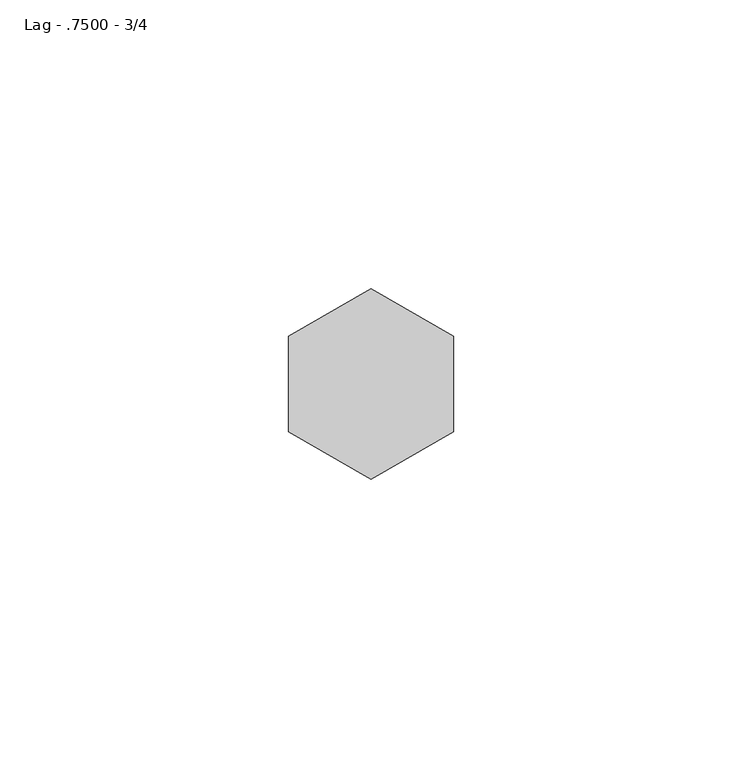
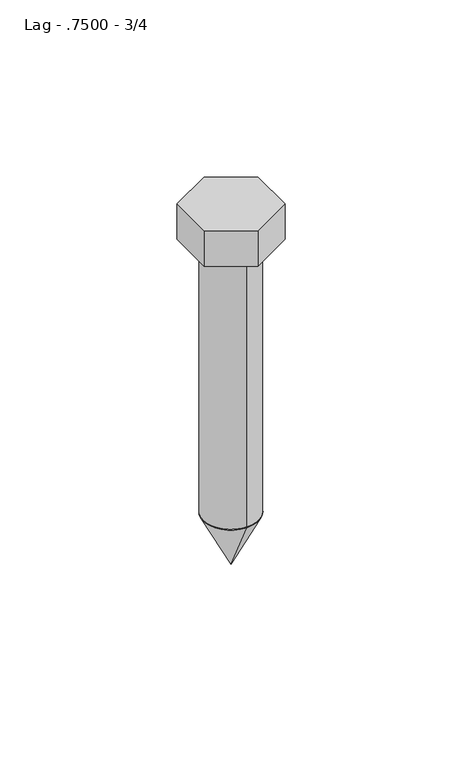
"""IFC4 building model written with IfcOpenShell, lengths in millimetres: fastener geometry, 060523 - W_P_C - Fastenings - Generic : Lag - .7500 - 3/4."""

from ifc_helpers import new_model, si_unit, point, frame, origin, origin_with_axes, origin_2d, place, context, project, spatial, polyline, circle_curve, trimmed, segment, composite_curve, outline, extrude, source, transform, mapped, element, save
from ifc_brep_helpers import plane_surface, revolved_surface, advanced_brep


def lag_7500_3_4_71b2816c(model_context):
    return source(origin(), model_context, "Body", "SolidModel", [
        advanced_brep(
        [(0.0, -9.7730469, -101.6), (0.0, 9.7730469, -101.6), (0.0, 0.0, -101.6), (0.0, 0.0, -121.1460937)],
        [
            (0, 1, circle_curve(frame((0.0, 0.0, -101.6), z_axis=(0.0, 0.0, 1.0), x_axis=(0.0, 1.0, 0.0)), 9.7730469)),
            (1, 2),
            (2, 0),
            (1, 0, circle_curve(frame((0.0, 0.0, -101.6), z_axis=(0.0, 0.0, 1.0), x_axis=(0.0, 1.0, 0.0)), 9.7730469)),
            (3, 1),
            (0, 3),
        ],
        [
            plane_surface(frame((0.0, 0.0, -101.6), z_axis=(0.0, 0.0, 1.0), x_axis=(0.0, 1.0, 0.0))),
            revolved_surface(polyline([(0.0, 9.7730469, -101.6), (0.0, 0.0, -121.1460937)]), (0.0, 0.0, -103.0840259), (0.0, 0.0, -1.0)),
        ],
        [
            (0, [[1, 2, 3]]),
            (0, [[4, -3, -2]]),
            (1, [[5, -1, 6]]),
            (1, [[-6, -4, -5]]),
        ],
    ),
        extrude(outline(polyline([(-14.2875, 8.248892), (0.0, 16.4977839), (14.2875, 8.248892), (14.2875, -8.248892), (0.0, -16.4977839), (-14.2875, -8.248892), (-14.2875, 8.248892)])), origin_with_axes(), (0.0, 0.0, 1.0), 13.2953125),
        extrude(outline(composite_curve([segment(trimmed(circle_curve(origin_2d(), 9.7730469), [point((0.0, -9.7730469))], [point((0.0, 9.7730469))], False, "CARTESIAN"), True, "CONTINUOUS"), segment(trimmed(circle_curve(origin_2d(), 9.7730469), [point((0.0, 9.7730469))], [point((0.0, -9.7730469))], False, "CARTESIAN"), True, "CONTINUOUS")], self_intersect=False)), frame((0.0, 0.0, -101.6), z_axis=(0.0, 0.0, 1.0), x_axis=(1.0, 0.0, 0.0)), (0.0, 0.0, 1.0), 101.6),
    ])


if __name__ == "__main__":
    model = new_model("IFC4")
    model_context = context("Model", 3, world=origin())
    ifc_project = project(units=[si_unit("LENGTHUNIT", "METRE", prefix="MILLI")], contexts=[model_context])
    site = spatial("IfcSite", under=ifc_project)
    building = spatial("IfcBuilding", under=site)
    placement = place(None, origin())
    lag_7500_3_4_shape = lag_7500_3_4_71b2816c(model_context)
    element("IfcFastener", 1, ObjectType="060523 - W_P_C - Fastenings - Generic : Lag - .7500 - 3/4", at=placement, inside=building, context=model_context, shape_type="MappedRepresentation", body=[
        mapped(lag_7500_3_4_shape, transform((0.0, 0.0, 0.0), x_axis=(1.0, 0.0, 0.0), y_axis=(0.0, 1.0, 0.0), z_axis=(0.0, 0.0, 1.0))),
    ])
    save(model, "model.ifc")

# Revit data of these elements
# Type "060523 - W_P_C - Fastenings - Generic : Lag - .7500 - 3/4"
#   Washer_Thickness = 0' - 0.17448"
#   Washer Radius = 0' - 0.9082"
#   Washer Offset - Head = 0' - 0"
#   Washer Offset = 0' - 0"
#   Thickness_of_Substrate [instance default] = 0' - 1"
#   Side = 0' - 0.65039"
#   Radius = 0' - 0.38477"
#   Length [instance default] = 0' - 4"
#   Head Size = 0' - 1 1/8"
#   Head Radius = 0' - 0 9/16"
#   Head Height = 0' - 0 67/128"
#   Double Diameter = 0' - 1 69/128"
#   Diameter = 0' - 0 197/256"
#   Default Elevation = 4' - 0"
#   Washer_Nut_Visibility = no
#   Washer_Head_Visibility = no
#   Round_Head_Visibility = no
#   Point Visibility = yes
#   Nut_Visibility = no
#   Hex_Head_Visiblilty = yes
#   Washer Material = none
#   Bolt Material (Size) = AT SILL - FASTENER AT 24" O.C.
# Element 1 (IfcFastener, "060523 - W_P_C - Fastenings - Generic : Lag - .7500 - 3/4")
#   Materials on its faces: "AT SILL - FASTENER AT 24\" O.C."
# Materials
#   "AT SILL - FASTENER AT 24\" O.C.": class "Generic", colour RGB 120 120 120, transparency 0, Cost = 0
